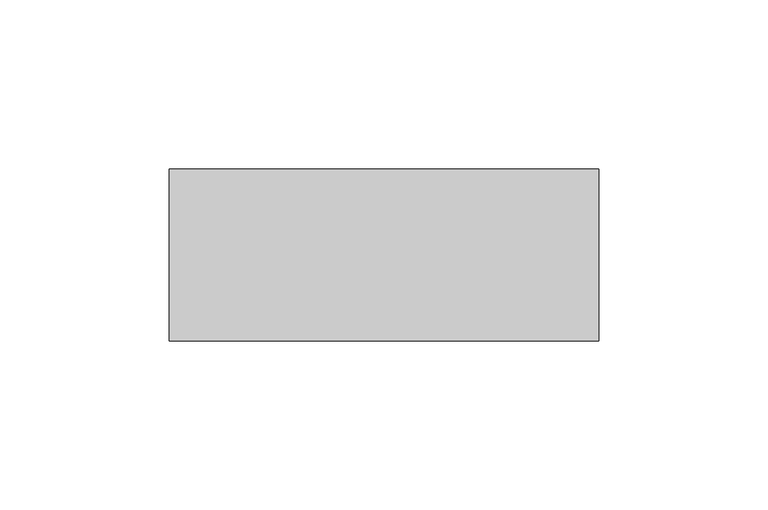
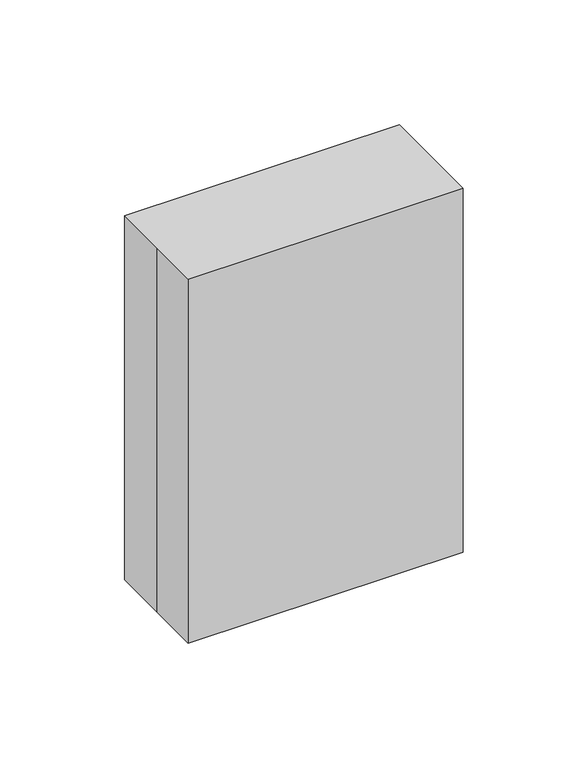
"""IFC4 building model written with IfcOpenShell, lengths in millimetres: proxy geometry, D4590 - Chisel, Dental, Pneumatic : D4590 - Chisel, Dental, Pneumatic."""

import ifcopenshell
import ifcopenshell.guid

model = None  # the IFC model being written
_history = None  # IfcOwnerHistory: only IFC2X3 demands one
_inside = {}  # id of a spatial element -> (the spatial element, [elements in it])
_under = {}  # id of a project, library or spatial element -> (it, [spatial elements below it])
_declared = {}  # id of a project -> (the project, [libraries it declares])
_typed = {}  # id of a type object -> (the type object, [elements of that type])
_made_of = {}  # id of a material, layer set ... -> (it, [elements and type objects made of it])


def new_model(schema):
    """Start an empty IFC model of exactly this schema.

    Asked for "IFC4X3", IfcOpenShell would pick the latest addendum, in which some entities
    have other attributes; the version numbers below select the first issue.
    IFC2X3 requires an IfcOwnerHistory on every rooted entity: one is made here for all.
    """
    global model, _history
    if schema == "IFC4X3":
        model = ifcopenshell.file(schema_version=(4, 3, 0, 0))
    else:
        model = ifcopenshell.file(schema=schema)
    _inside.clear()
    _under.clear()
    _declared.clear()
    _typed.clear()
    _made_of.clear()
    _history = None
    if model.schema == "IFC2X3":
        org = make("IfcOrganization", Name="unknown")
        user = make(
            "IfcPersonAndOrganization",
            ThePerson=make("IfcPerson", FamilyName="unknown"),
            TheOrganization=org,
        )
        app = make(
            "IfcApplication",
            ApplicationDeveloper=org,
            Version="unknown",
            ApplicationFullName="unknown",
            ApplicationIdentifier="unknown",
        )
        _history = make(
            "IfcOwnerHistory",
            OwningUser=user,
            OwningApplication=app,
            ChangeAction="ADDED",
            CreationDate=0,
        )
    return model


def make(cls, **values):
    """One entity of the class cls with the attributes given. An attribute that is None is left unset."""
    return model.create_entity(
        cls, **{name: value for name, value in values.items() if value is not None}
    )


def rooted(cls, **values):
    """An entity with a GlobalId (a new one), such as an element, a storey or a relation."""
    return make(cls, GlobalId=ifcopenshell.guid.new(), OwnerHistory=_history, **values)


def si_unit(unit_type, name, prefix=None):
    """IfcSIUnit, for example si_unit("LENGTHUNIT", "METRE", prefix="MILLI")."""
    return make("IfcSIUnit", UnitType=unit_type, Prefix=prefix, Name=name)


def assignment(units):
    """IfcUnitAssignment: the units of a project."""
    return None if units is None else make("IfcUnitAssignment", Units=units)


def point(xyz):
    """IfcCartesianPoint."""
    return None if xyz is None else make("IfcCartesianPoint", Coordinates=xyz)


def direction(xyz):
    """IfcDirection."""
    return None if xyz is None else make("IfcDirection", DirectionRatios=xyz)


def frame(location, z_axis=None, x_axis=None):
    """IfcAxis2Placement3D, a coordinate frame: its origin and axes. An axis left out is left unset."""
    return make(
        "IfcAxis2Placement3D",
        Location=point(location),
        Axis=direction(z_axis),
        RefDirection=direction(x_axis),
    )


def origin():
    """The frame at (0, 0, 0) with its axes left unset."""
    return frame((0.0, 0.0, 0.0))


def origin_with_axes():
    """The frame at (0, 0, 0) with the z axis (0, 0, 1) and the x axis (1, 0, 0) written out."""
    return frame((0.0, 0.0, 0.0), z_axis=(0.0, 0.0, 1.0), x_axis=(1.0, 0.0, 0.0))


def place(relative_to, where):
    """IfcLocalPlacement: puts the frame where relative to a parent placement (None: the world)."""
    return make(
        "IfcLocalPlacement", PlacementRelTo=relative_to, RelativePlacement=where
    )


def context(
    kind, dimensions, precision=None, world=None, true_north=None, identifier=None
):
    """IfcGeometricRepresentationContext, for example the 3D "Model" context."""
    return make(
        "IfcGeometricRepresentationContext",
        ContextIdentifier=identifier,
        ContextType=kind,
        CoordinateSpaceDimension=dimensions,
        Precision=precision,
        WorldCoordinateSystem=world,
        TrueNorth=true_north,
    )


def project(units=None, contexts=None):
    """IfcProject with its units and contexts."""
    return rooted(
        "IfcProject",
        Name="project",
        RepresentationContexts=contexts,
        UnitsInContext=assignment(units),
    )


def spatial(cls, under=None, at=None, **own):
    """A site, building, storey or space (cls), placed at a placement, below another one or the project."""
    s = rooted(cls, ObjectPlacement=at, **own)
    if under is not None:
        _under.setdefault(under.id(), (under, []))[1].append(s)
    return s


def polyline(points):
    """IfcPolyline through the points."""
    return make("IfcPolyline", Points=[point(p) for p in points])


def outline(outer, holes=None, kind="AREA"):
    """IfcArbitraryClosedProfileDef: a profile drawn as a closed curve; with holes, ...WithVoids."""
    if holes is None:
        return make("IfcArbitraryClosedProfileDef", ProfileType=kind, OuterCurve=outer)
    return make(
        "IfcArbitraryProfileDefWithVoids",
        ProfileType=kind,
        OuterCurve=outer,
        InnerCurves=holes,
    )


def extrude(swept, where, along, depth):
    """IfcExtrudedAreaSolid: the profile swept, set in the frame where, extruded along a direction by depth."""
    return make(
        "IfcExtrudedAreaSolid",
        SweptArea=swept,
        Position=where,
        ExtrudedDirection=direction(along),
        Depth=depth,
    )


def shape(context_of_items, identifier, shape_type, items):
    """IfcShapeRepresentation: the items that make up one representation, for example the "Body"."""
    return make(
        "IfcShapeRepresentation",
        ContextOfItems=context_of_items,
        RepresentationIdentifier=identifier,
        RepresentationType=shape_type,
        Items=items,
    )


def source(mapping_origin, context_of_items, identifier, shape_type, items):
    """IfcRepresentationMap: a shape defined once, which mapped items show again and again."""
    return make(
        "IfcRepresentationMap",
        MappingOrigin=mapping_origin,
        MappedRepresentation=shape(context_of_items, identifier, shape_type, items),
    )


def transform(
    local_origin,
    x_axis=None,
    y_axis=None,
    z_axis=None,
    scale=None,
    scale2=None,
    scale3=None,
    uniform=True,
):
    """IfcCartesianTransformationOperator3D, or its non-uniform kind. x_axis, y_axis, z_axis: its Axis1, 2, 3."""
    if uniform:
        return make(
            "IfcCartesianTransformationOperator3D",
            Axis1=direction(x_axis),
            Axis2=direction(y_axis),
            LocalOrigin=point(local_origin),
            Scale=scale,
            Axis3=direction(z_axis),
        )
    return make(
        "IfcCartesianTransformationOperator3DnonUniform",
        Axis1=direction(x_axis),
        Axis2=direction(y_axis),
        LocalOrigin=point(local_origin),
        Scale=scale,
        Axis3=direction(z_axis),
        Scale2=scale2,
        Scale3=scale3,
    )


def mapped(mapping_source, mapping_target):
    """IfcMappedItem: shows the shape of a source again, moved by a transform."""
    return make(
        "IfcMappedItem", MappingSource=mapping_source, MappingTarget=mapping_target
    )


def made_of(thing, what):
    """Note that an element or type object is made of a material, layer set ...; save() writes the relation."""
    if what is not None:
        _made_of.setdefault(what.id(), (what, []))[1].append(thing)
    return thing


def element(
    cls,
    number,
    at=None,
    inside=None,
    cuts=None,
    type_object=None,
    material=None,
    context=None,
    identifier="Body",
    shape_type=None,
    held_by="IfcProductDefinitionShape",
    body=None,
    shapes=None,
    **own,
):
    """One element of the class cls, such as IfcWall. Its Tag is "e" and its number.

    at: its placement. inside: the storey or other place that contains it. cuts: it is an
    opening in that element (IfcRelVoidsElement). A single representation is given by context,
    identifier, shape_type and body (its items); several are given by shapes. held_by: the class
    of the entity that holds the representations. save() writes the other relations.
    """
    e = rooted(cls, Tag="e%d" % number, ObjectPlacement=at, **own)
    if body is not None:
        shapes = [shape(context, identifier, shape_type, body)]
    if shapes is not None:
        e.Representation = make(held_by, Representations=shapes)
    if inside is not None:
        _inside.setdefault(inside.id(), (inside, []))[1].append(e)
    if cuts is not None:
        rooted(
            "IfcRelVoidsElement", RelatingBuildingElement=cuts, RelatedOpeningElement=e
        )
    if type_object is not None:
        _typed.setdefault(type_object.id(), (type_object, []))[1].append(e)
    return made_of(e, material)


def aggregate(whole, parts):
    """IfcRelAggregates: a whole, such as a stair, and the parts it consists of."""
    return rooted("IfcRelAggregates", RelatingObject=whole, RelatedObjects=parts)


def save(model, path):
    """Write the relations noted so far, then the file.

    IfcRelAggregates (storeys below a building ...), IfcRelContainedInSpatialStructure (elements
    in a storey), IfcRelDefinesByType, IfcRelAssociatesMaterial and IfcRelDeclares: one each for
    every whole, place, type object, material and project.
    """
    for whole, parts in _under.values():
        aggregate(whole, parts)
    for where, things in _inside.values():
        rooted(
            "IfcRelContainedInSpatialStructure",
            RelatedElements=things,
            RelatingStructure=where,
        )
    for kind, things in _typed.values():
        rooted("IfcRelDefinesByType", RelatedObjects=things, RelatingType=kind)
    for what, things in _made_of.values():
        rooted("IfcRelAssociatesMaterial", RelatedObjects=things, RelatingMaterial=what)
    for by, libraries in _declared.values():
        rooted("IfcRelDeclares", RelatingContext=by, RelatedDefinitions=libraries)
    model.write(path)


def specialty_equipment_db762eca(model_context):
    return source(origin(), model_context, "Body", "SweptSolid", [
        extrude(outline(polyline([(57.9280548, 17.7620366), (57.9280548, -20.3379634), (-56.3719452, -20.3379634), (-56.3719452, 17.7620366), (57.9280548, 17.7620366)])), origin_with_axes(), (0.0, 0.0, 1.0), 165.1),
        extrude(outline(polyline([(-63.5, 25.4), (63.5, 25.4), (63.5, -25.4), (-63.5, -25.4), (-63.5, 0.0), (-63.5, 25.4)])), origin_with_axes(), (0.0, 0.0, 1.0), 177.8),
    ])


if __name__ == "__main__":
    model = new_model("IFC4")
    model_context = context("Model", 3, world=origin())
    ifc_project = project(units=[si_unit("LENGTHUNIT", "METRE", prefix="MILLI")], contexts=[model_context])
    site = spatial("IfcSite", under=ifc_project)
    building = spatial("IfcBuilding", under=site)
    placement = place(None, origin())
    specialty_equipment_shape = specialty_equipment_db762eca(model_context)
    element("IfcBuildingElementProxy", 1, Name="D4590 - Chisel, Dental, Pneumatic : D4590 - Chisel, Dental, Pneumatic", ObjectType="D4590 - Chisel, Dental, Pneumatic : D4590 - Chisel, Dental, Pneumatic", at=placement, inside=building, context=model_context, shape_type="MappedRepresentation", body=[
        mapped(specialty_equipment_shape, transform((0.0, 0.0, 0.0), x_axis=(1.0, 0.0, 0.0), y_axis=(0.0, 1.0, 0.0), z_axis=(0.0, 0.0, 1.0))),
    ])
    save(model, "model.ifc")

# Revit data of these elements
# Type "D4590 - Chisel, Dental, Pneumatic : D4590 - Chisel, Dental, Pneumatic"
#   Watts2 = "0"
#   Watts1 = "0"
#   Unit_Issue = "EA"
#   UTIL_6_Misc = "-"
#   UTIL_5_NonMedGas = "-"
#   UTIL_4_MiscGas = "-"
#   UTIL_3_MedGas = "D"
#   UTIL_2_Elec = "-"
#   UTIL_1_WaterDrain = "-"
#   Nomenclature = "Chisel, Dental, Pneumatic"
#   NSN = "6520"
#   Location [instance default] = ""
#   JSN = "D4590"
#   Fund_Source_VA = "-"
#   Fund_Source_Navy = "-"
#   Fund_Source_Army = "-"
#   Fund_Source_AF = "-"
#   ELEC_Volts2 = "0"
#   ELEC_Volts1 = "0"
#   ELEC_Phase2 = "0"
#   ELEC_Phase1 = "0"
#   ELEC_HertzSwitch = "0"
#   ELEC_HertzDependent = "0"
#   ELEC_Hertz = "0"
#   ELEC_Amps2 = "0"
#   ELEC_Amps1 = "0"
#   DetailDescription = "Pneumatic dental chisel. The chisel is used in a dental laboratory for prosthodontic appliance deflasking. Several different chisel tips are available. Some units require an oil atomizer for proper operation."
#   CAT_VA = "C"
#   CAT_Navy = "C"
#   CAT_IHS = "-"
#   CAT_Army = "C"
#   CAT_AF = "C"
#   BTUperhour = "0"
#   Weight_IP = 1
#   DIM_Width_IP = 0' - 5"
#   DIM_Height_IP = 0' - 7"
#   DIM_Depth_IP = 0' - 2"
# Element 1 (IfcBuildingElementProxy, "D4590 - Chisel, Dental, Pneumatic : D4590 - Chisel, Dental, Pneumatic")
#   Location = "DNPL2"
#   Materials on its faces: "EquipSpace"
# Materials
#   "EquipSpace": class "Unassigned", colour RGB 221 217 195, transparency 0.5
